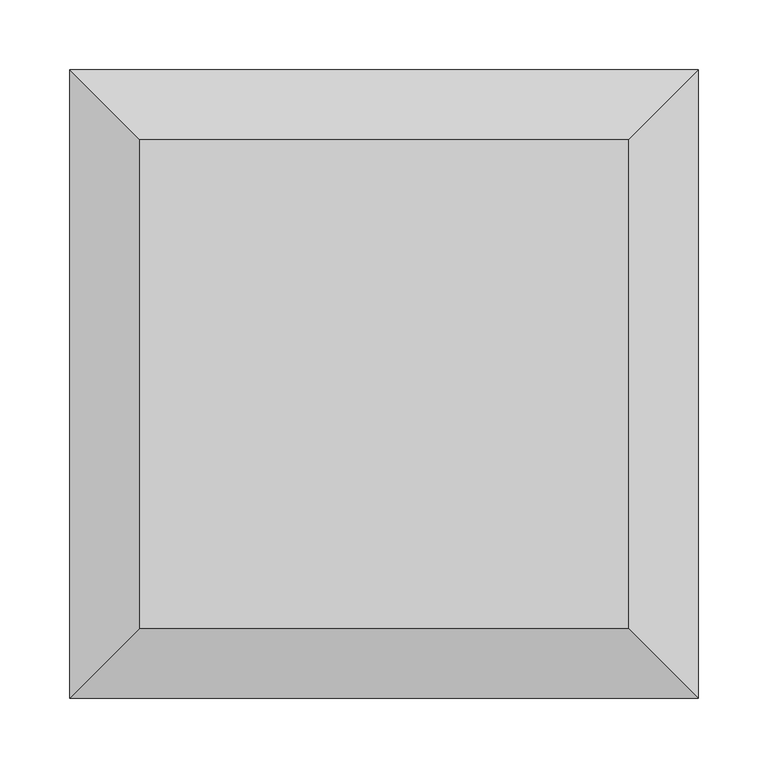
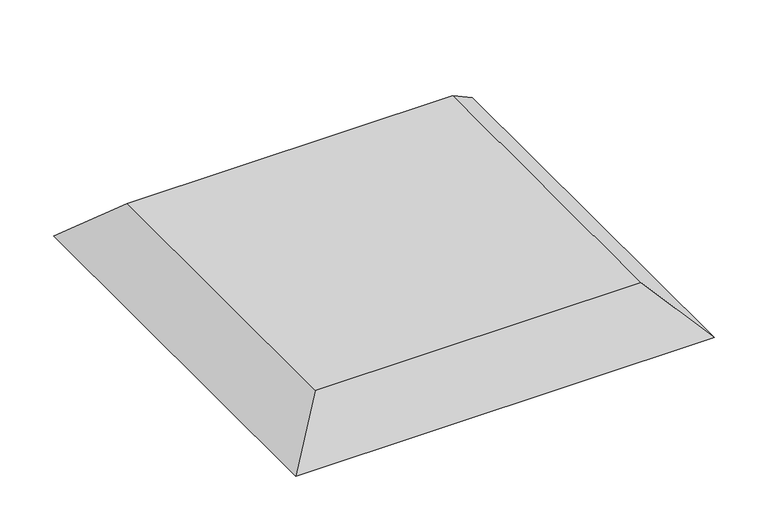
"""IFC4 building model written with IfcOpenShell, lengths in millimetres: proxy geometry, 그라우트19 : 그라우트."""

from ifc_helpers import new_model, si_unit, origin, place, context, project, spatial, faceted_brep, source, transform, mapped, element, save


def generic_models_49ee4eb4(model_context):
    return source(origin(), model_context, "Body", "Brep", [
        faceted_brep([(25169.0, 25924.5208589, 743.9720055), (24819.0, 25924.5208589, 743.9720055), (24819.0, 25574.5208589, 743.9720055), (25169.0, 25574.5208589, 743.9720055), (25219.0, 25974.5208589, 693.9720055), (25219.0, 25524.5208589, 693.9720055), (24769.0, 25524.5208589, 693.9720055), (24769.0, 25974.5208589, 693.9720055)], [[[0, 1, 2, 3]], [[4, 5, 6, 7]], [[4, 7, 1, 0]], [[7, 6, 2, 1]], [[6, 5, 3, 2]], [[5, 4, 0, 3]]]),
    ])


if __name__ == "__main__":
    model = new_model("IFC4")
    model_context = context("Model", 3, world=origin())
    ifc_project = project(units=[si_unit("LENGTHUNIT", "METRE", prefix="MILLI")], contexts=[model_context])
    site = spatial("IfcSite", under=ifc_project)
    building = spatial("IfcBuilding", under=site)
    placement = place(None, origin())
    generic_models_shape = generic_models_49ee4eb4(model_context)
    element("IfcBuildingElementProxy", 1, Name="그라우트19 : 그라우트", ObjectType="그라우트19 : 그라우트", at=placement, inside=building, context=model_context, shape_type="MappedRepresentation", body=[
        mapped(generic_models_shape, transform((0.0, 0.0, 0.0), x_axis=(1.0, 0.0, 0.0), y_axis=(0.0, 1.0, 0.0), z_axis=(0.0, 0.0, 1.0))),
    ])
    save(model, "model.ifc")
